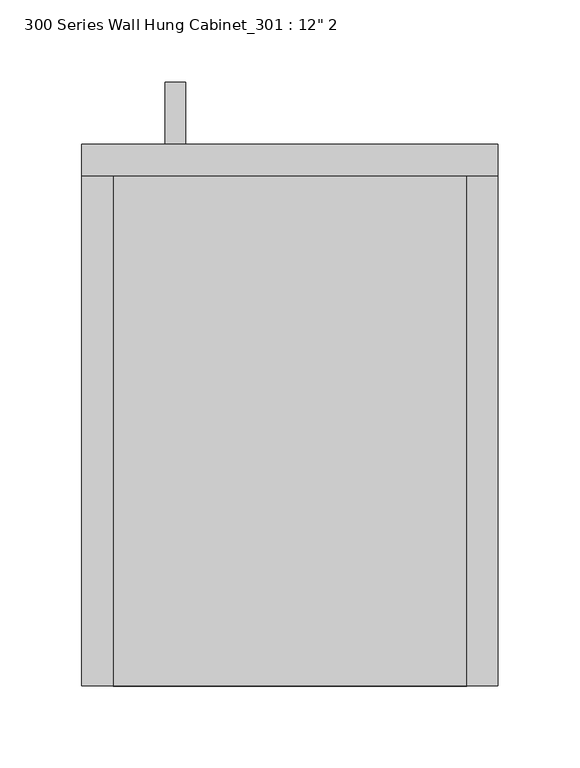
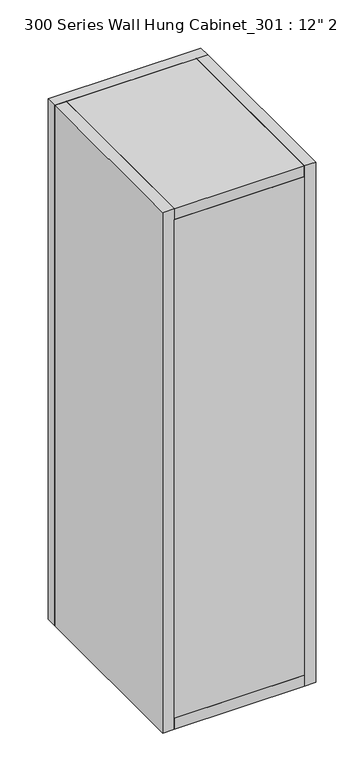
"""IFC4 building model written with IfcOpenShell, lengths in millimetres: furniture geometry."""

import ifcopenshell
import ifcopenshell.guid

model = None  # the IFC model being written
_history = None  # IfcOwnerHistory: only IFC2X3 demands one
_inside = {}  # id of a spatial element -> (the spatial element, [elements in it])
_under = {}  # id of a project, library or spatial element -> (it, [spatial elements below it])
_declared = {}  # id of a project -> (the project, [libraries it declares])
_typed = {}  # id of a type object -> (the type object, [elements of that type])
_made_of = {}  # id of a material, layer set ... -> (it, [elements and type objects made of it])


def new_model(schema):
    """Start an empty IFC model of exactly this schema.

    Asked for "IFC4X3", IfcOpenShell would pick the latest addendum, in which some entities
    have other attributes; the version numbers below select the first issue.
    IFC2X3 requires an IfcOwnerHistory on every rooted entity: one is made here for all.
    """
    global model, _history
    if schema == "IFC4X3":
        model = ifcopenshell.file(schema_version=(4, 3, 0, 0))
    else:
        model = ifcopenshell.file(schema=schema)
    _inside.clear()
    _under.clear()
    _declared.clear()
    _typed.clear()
    _made_of.clear()
    _history = None
    if model.schema == "IFC2X3":
        org = make("IfcOrganization", Name="unknown")
        user = make(
            "IfcPersonAndOrganization",
            ThePerson=make("IfcPerson", FamilyName="unknown"),
            TheOrganization=org,
        )
        app = make(
            "IfcApplication",
            ApplicationDeveloper=org,
            Version="unknown",
            ApplicationFullName="unknown",
            ApplicationIdentifier="unknown",
        )
        _history = make(
            "IfcOwnerHistory",
            OwningUser=user,
            OwningApplication=app,
            ChangeAction="ADDED",
            CreationDate=0,
        )
    return model


def make(cls, **values):
    """One entity of the class cls with the attributes given. An attribute that is None is left unset."""
    return model.create_entity(
        cls, **{name: value for name, value in values.items() if value is not None}
    )


def rooted(cls, **values):
    """An entity with a GlobalId (a new one), such as an element, a storey or a relation."""
    return make(cls, GlobalId=ifcopenshell.guid.new(), OwnerHistory=_history, **values)


def si_unit(unit_type, name, prefix=None):
    """IfcSIUnit, for example si_unit("LENGTHUNIT", "METRE", prefix="MILLI")."""
    return make("IfcSIUnit", UnitType=unit_type, Prefix=prefix, Name=name)


def assignment(units):
    """IfcUnitAssignment: the units of a project."""
    return None if units is None else make("IfcUnitAssignment", Units=units)


def point(xyz):
    """IfcCartesianPoint."""
    return None if xyz is None else make("IfcCartesianPoint", Coordinates=xyz)


def direction(xyz):
    """IfcDirection."""
    return None if xyz is None else make("IfcDirection", DirectionRatios=xyz)


def frame(location, z_axis=None, x_axis=None):
    """IfcAxis2Placement3D, a coordinate frame: its origin and axes. An axis left out is left unset."""
    return make(
        "IfcAxis2Placement3D",
        Location=point(location),
        Axis=direction(z_axis),
        RefDirection=direction(x_axis),
    )


def origin():
    """The frame at (0, 0, 0) with its axes left unset."""
    return frame((0.0, 0.0, 0.0))


def place(relative_to, where):
    """IfcLocalPlacement: puts the frame where relative to a parent placement (None: the world)."""
    return make(
        "IfcLocalPlacement", PlacementRelTo=relative_to, RelativePlacement=where
    )


def context(
    kind, dimensions, precision=None, world=None, true_north=None, identifier=None
):
    """IfcGeometricRepresentationContext, for example the 3D "Model" context."""
    return make(
        "IfcGeometricRepresentationContext",
        ContextIdentifier=identifier,
        ContextType=kind,
        CoordinateSpaceDimension=dimensions,
        Precision=precision,
        WorldCoordinateSystem=world,
        TrueNorth=true_north,
    )


def project(units=None, contexts=None):
    """IfcProject with its units and contexts."""
    return rooted(
        "IfcProject",
        Name="project",
        RepresentationContexts=contexts,
        UnitsInContext=assignment(units),
    )


def spatial(cls, under=None, at=None, **own):
    """A site, building, storey or space (cls), placed at a placement, below another one or the project."""
    s = rooted(cls, ObjectPlacement=at, **own)
    if under is not None:
        _under.setdefault(under.id(), (under, []))[1].append(s)
    return s


def polyline(points):
    """IfcPolyline through the points."""
    return make("IfcPolyline", Points=[point(p) for p in points])


def outline(outer, holes=None, kind="AREA"):
    """IfcArbitraryClosedProfileDef: a profile drawn as a closed curve; with holes, ...WithVoids."""
    if holes is None:
        return make("IfcArbitraryClosedProfileDef", ProfileType=kind, OuterCurve=outer)
    return make(
        "IfcArbitraryProfileDefWithVoids",
        ProfileType=kind,
        OuterCurve=outer,
        InnerCurves=holes,
    )


def extrude(swept, where, along, depth):
    """IfcExtrudedAreaSolid: the profile swept, set in the frame where, extruded along a direction by depth."""
    return make(
        "IfcExtrudedAreaSolid",
        SweptArea=swept,
        Position=where,
        ExtrudedDirection=direction(along),
        Depth=depth,
    )


def shape(context_of_items, identifier, shape_type, items):
    """IfcShapeRepresentation: the items that make up one representation, for example the "Body"."""
    return make(
        "IfcShapeRepresentation",
        ContextOfItems=context_of_items,
        RepresentationIdentifier=identifier,
        RepresentationType=shape_type,
        Items=items,
    )


def source(mapping_origin, context_of_items, identifier, shape_type, items):
    """IfcRepresentationMap: a shape defined once, which mapped items show again and again."""
    return make(
        "IfcRepresentationMap",
        MappingOrigin=mapping_origin,
        MappedRepresentation=shape(context_of_items, identifier, shape_type, items),
    )


def transform(
    local_origin,
    x_axis=None,
    y_axis=None,
    z_axis=None,
    scale=None,
    scale2=None,
    scale3=None,
    uniform=True,
):
    """IfcCartesianTransformationOperator3D, or its non-uniform kind. x_axis, y_axis, z_axis: its Axis1, 2, 3."""
    if uniform:
        return make(
            "IfcCartesianTransformationOperator3D",
            Axis1=direction(x_axis),
            Axis2=direction(y_axis),
            LocalOrigin=point(local_origin),
            Scale=scale,
            Axis3=direction(z_axis),
        )
    return make(
        "IfcCartesianTransformationOperator3DnonUniform",
        Axis1=direction(x_axis),
        Axis2=direction(y_axis),
        LocalOrigin=point(local_origin),
        Scale=scale,
        Axis3=direction(z_axis),
        Scale2=scale2,
        Scale3=scale3,
    )


def mapped(mapping_source, mapping_target):
    """IfcMappedItem: shows the shape of a source again, moved by a transform."""
    return make(
        "IfcMappedItem", MappingSource=mapping_source, MappingTarget=mapping_target
    )


def made_of(thing, what):
    """Note that an element or type object is made of a material, layer set ...; save() writes the relation."""
    if what is not None:
        _made_of.setdefault(what.id(), (what, []))[1].append(thing)
    return thing


def element(
    cls,
    number,
    at=None,
    inside=None,
    cuts=None,
    type_object=None,
    material=None,
    context=None,
    identifier="Body",
    shape_type=None,
    held_by="IfcProductDefinitionShape",
    body=None,
    shapes=None,
    **own,
):
    """One element of the class cls, such as IfcWall. Its Tag is "e" and its number.

    at: its placement. inside: the storey or other place that contains it. cuts: it is an
    opening in that element (IfcRelVoidsElement). A single representation is given by context,
    identifier, shape_type and body (its items); several are given by shapes. held_by: the class
    of the entity that holds the representations. save() writes the other relations.
    """
    e = rooted(cls, Tag="e%d" % number, ObjectPlacement=at, **own)
    if body is not None:
        shapes = [shape(context, identifier, shape_type, body)]
    if shapes is not None:
        e.Representation = make(held_by, Representations=shapes)
    if inside is not None:
        _inside.setdefault(inside.id(), (inside, []))[1].append(e)
    if cuts is not None:
        rooted(
            "IfcRelVoidsElement", RelatingBuildingElement=cuts, RelatedOpeningElement=e
        )
    if type_object is not None:
        _typed.setdefault(type_object.id(), (type_object, []))[1].append(e)
    return made_of(e, material)


def aggregate(whole, parts):
    """IfcRelAggregates: a whole, such as a stair, and the parts it consists of."""
    return rooted("IfcRelAggregates", RelatingObject=whole, RelatedObjects=parts)


def save(model, path):
    """Write the relations noted so far, then the file.

    IfcRelAggregates (storeys below a building ...), IfcRelContainedInSpatialStructure (elements
    in a storey), IfcRelDefinesByType, IfcRelAssociatesMaterial and IfcRelDeclares: one each for
    every whole, place, type object, material and project.
    """
    for whole, parts in _under.values():
        aggregate(whole, parts)
    for where, things in _inside.values():
        rooted(
            "IfcRelContainedInSpatialStructure",
            RelatedElements=things,
            RelatingStructure=where,
        )
    for kind, things in _typed.values():
        rooted("IfcRelDefinesByType", RelatedObjects=things, RelatingType=kind)
    for what, things in _made_of.values():
        rooted("IfcRelAssociatesMaterial", RelatedObjects=things, RelatingMaterial=what)
    for by, libraries in _declared.values():
        rooted("IfcRelDeclares", RelatingContext=by, RelatedDefinitions=libraries)
    model.write(path)


def furniture_3e0bc3ae(model_context):
    return source(origin(), model_context, "Body", "SweptSolid", [
        extrude(outline(polyline([(390.525, 1352.5425373), (390.525, 1365.2121874), (428.6060937, 1365.2121874), (428.6060937, 1270.0), (390.525, 1270.0), (390.525, 1282.6696501), (415.9364436, 1282.6696501), (415.9364436, 1352.5425373), (390.525, 1352.5425373)])), frame((-76.2, 0.0, 0.0), z_axis=(1.0, 0.0, 0.0), x_axis=(0.0, 1.0, 0.0)), (0.0, 0.0, 1.0), 12.4065288),
        extrude(outline(polyline([(107.95, 371.475), (107.95, 60.325), (-107.95, 60.325), (-107.95, 371.475), (107.95, 371.475)])), frame((0.0, 0.0, 1219.2), z_axis=(0.0, 0.0, 1.0), x_axis=(1.0, 0.0, 0.0)), (0.0, 0.0, 1.0), 19.05),
        extrude(outline(polyline([(107.95, 60.325), (-107.95, 60.325), (-107.95, 79.375), (107.95, 79.375), (107.95, 60.325)])), frame((0.0, 0.0, 1238.25), z_axis=(0.0, 0.0, 1.0), x_axis=(1.0, 0.0, 0.0)), (0.0, 0.0, 1.0), 876.3),
        extrude(outline(polyline([(127.0, 371.475), (-127.0, 371.475), (-127.0, 390.525), (127.0, 390.525), (127.0, 371.475)])), frame((0.0, 0.0, 1219.2), z_axis=(0.0, 0.0, 1.0), x_axis=(1.0, 0.0, 0.0)), (0.0, 0.0, 1.0), 914.4),
        extrude(outline(polyline([(-127.0, 60.325), (-127.0, 371.475), (-107.95, 371.475), (-107.95, 60.325), (-127.0, 60.325)])), frame((0.0, 0.0, 1219.2), z_axis=(0.0, 0.0, 1.0), x_axis=(1.0, 0.0, 0.0)), (0.0, 0.0, 1.0), 914.4),
        extrude(outline(polyline([(107.95, 60.325), (107.95, 371.475), (127.0, 371.475), (127.0, 60.325), (107.95, 60.325)])), frame((0.0, 0.0, 1219.2), z_axis=(0.0, 0.0, 1.0), x_axis=(1.0, 0.0, 0.0)), (0.0, 0.0, 1.0), 914.4),
        extrude(outline(polyline([(107.95, 371.475), (107.95, 60.325), (-107.95, 60.325), (-107.95, 371.475), (107.95, 371.475)])), frame((0.0, 0.0, 2114.55), z_axis=(0.0, 0.0, 1.0), x_axis=(1.0, 0.0, 0.0)), (0.0, 0.0, 1.0), 19.05),
    ])


if __name__ == "__main__":
    model = new_model("IFC4")
    model_context = context("Model", 3, world=origin())
    ifc_project = project(units=[si_unit("LENGTHUNIT", "METRE", prefix="MILLI")], contexts=[model_context])
    site = spatial("IfcSite", under=ifc_project)
    building = spatial("IfcBuilding", under=site)
    placement = place(None, origin())
    furniture_shape = furniture_3e0bc3ae(model_context)
    element("IfcFurniture", 1, ObjectType="300 Series Wall Hung Cabinet_301 : 12\" 2", at=placement, inside=building, context=model_context, shape_type="MappedRepresentation", body=[
        mapped(furniture_shape, transform((0.0, 0.0, 0.0), x_axis=(1.0, 0.0, 0.0), y_axis=(0.0, 1.0, 0.0), z_axis=(0.0, 0.0, 1.0))),
    ])
    save(model, "model.ifc")

# Revit data of these elements
# Type "300 Series Wall Hung Cabinet_301 : 12\" 2"
#   URL = "www.wicnet.org/manual_sections.asp"
#   Model = "301"
#   Manufacturer = "Woodwork Institute"
#   Description = "Wall Hung Cabinet"
#   Content Creator URL = "www.AECcontent.com"
#   Content Creator = "AECcontent"
#   Assembly Code = "E2010200"
#   Width = 0' - 10"
#   Top of Cabinet = 7' - 0"
#   Height = 3' - 0"
#   Depth = 1' - 1"
#   Top Panel Material = none
#   Side Panel Material = none
#   Door Panel Material = none
#   Shelf Panel Material = none
# Element 1 (IfcFurniture, "300 Series Wall Hung Cabinet_301 : 12\" 2")
#   Materials on its faces: "CASEWORK"
# Materials
#   "CASEWORK": class "Generic", colour RGB 181 181 181, transparency 0, Cost = 0
